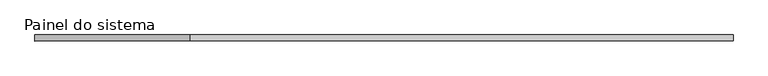
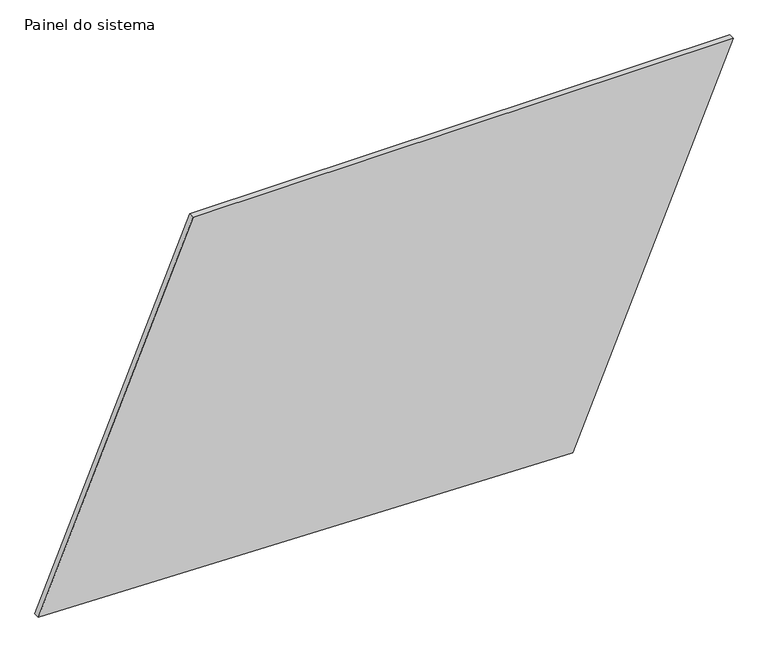
"""IFC4 building model written with IfcOpenShell, lengths in millimetres: plate geometry, Painel do sistema : Envidraçado."""

from ifc_helpers import new_model, si_unit, frame, origin, place, context, project, spatial, polyline, outline, extrude, source, transform, mapped, element, save


def painel_do_sistema_c7213802(model_context):
    return source(origin(), model_context, "Body", "SweptSolid", [
        extrude(outline(polyline([(54.9376383, -1438.2827715), (0.0, 774.6531006), (1581.6886998, 1438.2827715), (1581.6886998, -797.7033044), (54.9376383, -1438.2827715)])), frame((0.0, 24.5, 0.0), z_axis=(0.0, 1.0, 0.0), x_axis=(0.0, 0.0, 1.0)), (0.0, 0.0, 1.0), 25.0),
    ])


if __name__ == "__main__":
    model = new_model("IFC4")
    model_context = context("Model", 3, world=origin())
    ifc_project = project(units=[si_unit("LENGTHUNIT", "METRE", prefix="MILLI")], contexts=[model_context])
    site = spatial("IfcSite", under=ifc_project)
    building = spatial("IfcBuilding", under=site)
    placement = place(None, origin())
    painel_do_sistema_shape = painel_do_sistema_c7213802(model_context)
    element("IfcPlate", 1, ObjectType="Painel do sistema : Envidraçado", at=placement, inside=building, context=model_context, shape_type="MappedRepresentation", body=[
        mapped(painel_do_sistema_shape, transform((0.0, 0.0, 0.0), x_axis=(1.0, 0.0, 0.0), y_axis=(0.0, 1.0, 0.0), z_axis=(0.0, 0.0, 1.0))),
    ])
    save(model, "model.ifc")

# Revit data of these elements
# Type "Painel do sistema : Envidraçado"
#   Construction Type Id = "GSP4R"
#   Analytic Construction = "Vidraça única Pilkington 1/8 pol"
#   Visual Light Transmittance = 0.9
#   Solar Heat Gain Coefficient = 0.86
#   Heat Transfer Coefficient (U) = 6.7069 W/(m²·K)
# Element 1 (IfcPlate, "Painel do sistema : Envidraçado")
#   Materials on its faces: "Vidro"
# Materials
#   "Vidro": class "Vidro", colour RGB 0 128 192, transparency 0.9, Description = "Vidro de sílica", Cost = 0
